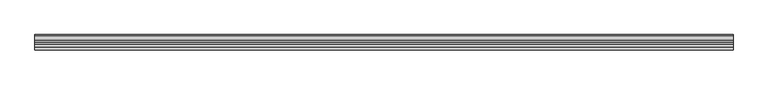
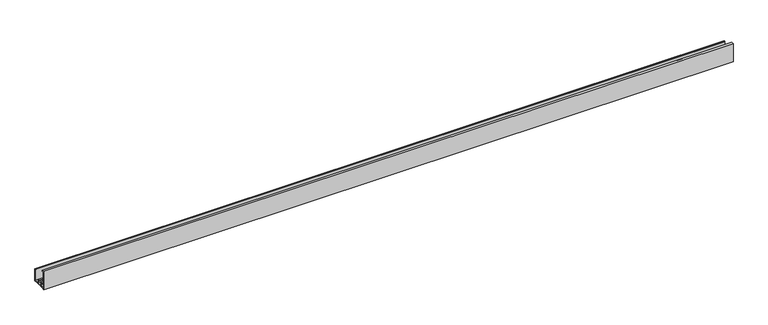
"""IFC4 building model written with IfcOpenShell, lengths in millimetres: proxy geometry, Generic Models 3:Generic Models 2:312240:Generic Models 2:312240 : Generic Models 3:Generic Models 2:312240:2 : Generic Models 3:Generic Models 2:312240:Generic Models 2:312240 : Generic Models 3:Generic Models 2:312240:300533."""

from ifc_helpers import new_model, si_unit, frame, origin, place, context, project, spatial, polyline, outline, extrude, source, transform, mapped, element, save


def generic_models_a0de8bba(model_context):
    return source(origin(), model_context, "Body", "SweptSolid", [
        extrude(outline(polyline([(-536487.197208, 8552.1457253), (-536487.197208, 8547.4482267), (-536489.1226234, 8547.4482267), (-536489.1226234, 8545.0669767), (-536487.197208, 8545.0669767), (-536487.197208, 8540.369478), (-536503.7494641, 8540.369478), (-536503.7494641, 8545.0669767), (-536501.8240487, 8545.0669767), (-536501.8240487, 8547.4482267), (-536503.7494641, 8547.4482267), (-536503.7494641, 8552.1457253), (-536487.197208, 8552.1457253)])), frame((591391.6367242, 0.0, 0.0), z_axis=(1.0, 0.0, 0.0), x_axis=(0.0, 1.0, 0.0)), (0.0, 0.0, 1.0), 2438.4),
        extrude(outline(polyline([(-536510.7868526, 8604.797603), (-536510.7868526, 8600.4102765), (-536512.3743526, 8600.4102765), (-536512.3743526, 8603.210103), (-536517.6457241, 8603.210103), (-536517.6457241, 8554.1301003), (-536499.9791516, 8554.1301003), (-536499.9791516, 8552.5426003), (-536504.1463391, 8552.5426003), (-536504.1463391, 8547.0513517), (-536502.2209237, 8547.0513517), (-536502.2209237, 8545.4638517), (-536504.1463391, 8545.4638517), (-536504.1463391, 8539.972603), (-536499.9791516, 8539.972603), (-536499.9791516, 8538.385103), (-536517.6457241, 8538.385103), (-536517.6457241, 8536.797603), (-536519.2332241, 8536.797603), (-536519.2332241, 8604.797603), (-536510.7868526, 8604.797603)]), holes=[polyline([(-536517.6457241, 8552.5426003), (-536517.6457241, 8539.972603), (-536505.7338391, 8539.972603), (-536505.7338391, 8552.5426003), (-536517.6457241, 8552.5426003)])]), frame((591391.6367242, 0.0, 0.0), z_axis=(1.0, 0.0, 0.0), x_axis=(0.0, 1.0, 0.0)), (0.0, 0.0, 1.0), 2438.4),
        extrude(outline(polyline([(-536466.8207241, 8536.797603), (-536466.8207241, 8538.385103), (-536490.9675205, 8538.385103), (-536490.9675205, 8539.972603), (-536486.800333, 8539.972603), (-536486.800333, 8545.4638517), (-536488.7257484, 8545.4638517), (-536488.7257484, 8547.0513517), (-536486.800333, 8547.0513517), (-536486.800333, 8552.5426003), (-536490.9675205, 8552.5426003), (-536490.9675205, 8554.1301003), (-536485.212833, 8554.1301003), (-536485.212833, 8539.972603), (-536466.8207241, 8539.972603), (-536466.8207241, 8581.2147905), (-536467.9483141, 8581.2147905), (-536467.9483141, 8582.8022905), (-536465.2332241, 8582.8022905), (-536465.2332241, 8536.797603), (-536466.8207241, 8536.797603)])), frame((591391.6367242, 0.0, 0.0), z_axis=(1.0, 0.0, 0.0), x_axis=(0.0, 1.0, 0.0)), (0.0, 0.0, 1.0), 2438.4),
    ])


if __name__ == "__main__":
    model = new_model("IFC4")
    model_context = context("Model", 3, world=origin())
    ifc_project = project(units=[si_unit("LENGTHUNIT", "METRE", prefix="MILLI")], contexts=[model_context])
    site = spatial("IfcSite", under=ifc_project)
    building = spatial("IfcBuilding", under=site)
    placement = place(None, origin())
    generic_models_shape = generic_models_a0de8bba(model_context)
    element("IfcBuildingElementProxy", 1, Name="Generic Models 3:Generic Models 2:312240:Generic Models 2:312240 : Generic Models 3:Generic Models 2:312240:2 : Generic Models 3:Generic Models 2:312240:Generic Models 2:312240 : Generic Models 3:Generic Models 2:312240:300533", ObjectType="Generic Models 3:Generic Models 2:312240:Generic Models 2:312240 : Generic Models 3:Generic Models 2:312240:2 : Generic Models 3:Generic Models 2:312240:Generic Models 2:312240 : Generic Models 3:Generic Models 2:312240:300533", at=placement, inside=building, context=model_context, shape_type="MappedRepresentation", body=[
        mapped(generic_models_shape, transform((0.0, 0.0, 0.0), x_axis=(1.0, 0.0, 0.0), y_axis=(0.0, 1.0, 0.0), z_axis=(0.0, 0.0, 1.0))),
    ])
    save(model, "model.ifc")

# Revit data of these elements
# Type "Generic Models 3:Generic Models 2:312240:Generic Models 2:312240 : Generic Models 3:Generic Models 2:312240:2 : Generic Models 3:Generic Models 2:312240:Generic Models 2:312240 : Generic Models 3:Generic Models 2:312240:300533"
#   NameOverride = "Generic Models 3:Generic Models 2:312240:Generic Models 2:312240 : Generic Models 3:Generic Models 2:312240:300533"
#   ObjectTypeOverride = "Generic Models 2:312240 : Generic Models 3:Generic Models 2:312240"
#   Reference = "Generic Models 2"
#   Tag = "300533"
# Element 1 (IfcBuildingElementProxy, "Generic Models 3:Generic Models 2:312240:Generic Models 2:312240 : Generic Models 3:Generic Models 2:312240:2 : Generic Models 3:Generic Models 2:312240:Generic Models 2:312240 : Generic Models 3:Generic Models 2:312240:300533")
#   Materials on its faces: "THERMAL BROKEN ALUMINUM STOREFRONT FOR POLYCARBONATE"
# Materials
#   "THERMAL BROKEN ALUMINUM STOREFRONT FOR POLYCARBONATE": class "Unassigned", colour RGB 244 244 244, transparency 0, Keynote = "M07611300.01", Cost = 0
